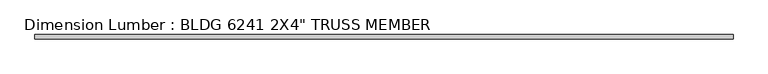
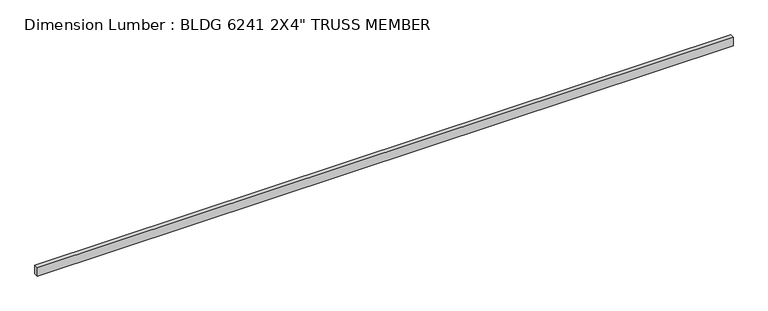
"""IFC4 building model written with IfcOpenShell, lengths in millimetres: beam geometry."""

from ifc_helpers import new_model, si_unit, frame, origin, place, context, project, spatial, polyline, outline, extrude, source, transform, mapped, element, save


def beam_0149d91d(model_context):
    return source(origin(), model_context, "Body", "SweptSolid", [
        extrude(outline(polyline([(4058.832951, 25.4), (4058.832951, -25.4), (-4033.432951, -25.4), (-4033.432951, 25.4), (4058.832951, 25.4)])), frame((0.0, 0.0, -50.8), z_axis=(0.0, 0.0, 1.0), x_axis=(1.0, 0.0, 0.0)), (0.0, 0.0, 1.0), 101.6),
    ])


if __name__ == "__main__":
    model = new_model("IFC4")
    model_context = context("Model", 3, world=origin())
    ifc_project = project(units=[si_unit("LENGTHUNIT", "METRE", prefix="MILLI")], contexts=[model_context])
    site = spatial("IfcSite", under=ifc_project)
    building = spatial("IfcBuilding", under=site)
    placement = place(None, origin())
    beam_shape = beam_0149d91d(model_context)
    element("IfcBeam", 1, ObjectType="Dimension Lumber : BLDG 6241 2X4\" TRUSS MEMBER", at=placement, inside=building, context=model_context, shape_type="MappedRepresentation", body=[
        mapped(beam_shape, transform((0.0, 0.0, 0.0), x_axis=(1.0, 0.0, 0.0), y_axis=(0.0, 1.0, 0.0), z_axis=(0.0, 0.0, 1.0))),
    ])
    save(model, "model.ifc")

# Revit data of these elements
# Type "Dimension Lumber : BLDG 6241 2X4\" TRUSS MEMBER"
#   Assembly Code = "B10"
#   A = 0.273472 SF
#   Length [instance default] = 5' - 0"
#   b = 0' - 2"
#   d = 0' - 4"
#   Structural Material [instance default] = Softwood, Lumber
# Element 1 (IfcBeam, "Dimension Lumber : BLDG 6241 2X4\" TRUSS MEMBER")
#   Materials on its faces: "Softwood, Lumber"
# Materials
#   "Softwood, Lumber": class "Wood", colour RGB 223 192 134, transparency 0, Description = "Pinus Echinata", Cost = 0
